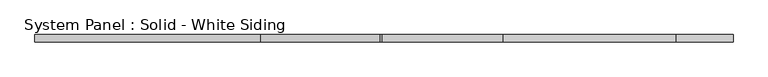
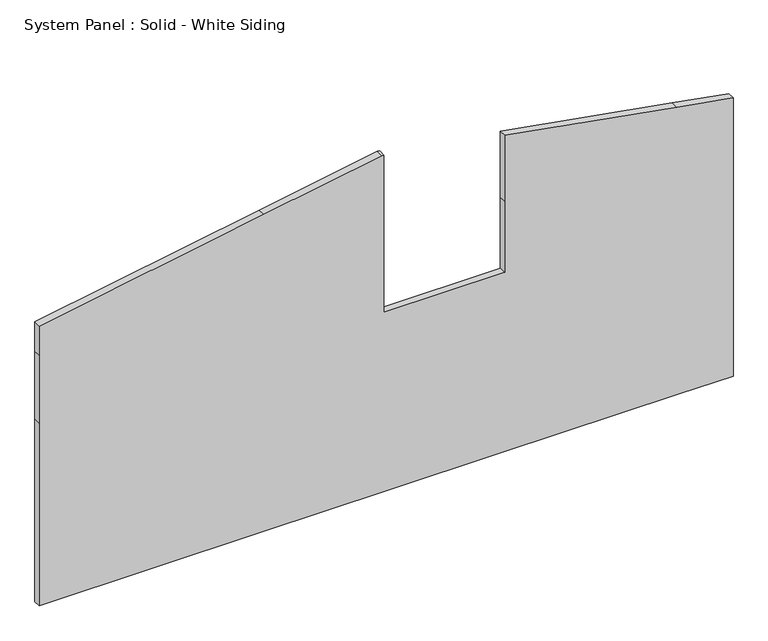
"""IFC4 building model written with IfcOpenShell, lengths in millimetres: plate geometry, System Panel : Solid - White Siding."""

from ifc_helpers import new_model, si_unit, frame, origin, place, context, project, spatial, polyline, outline, extrude, source, transform, mapped, element, save


def system_panel_solid_white_siding_d1a1bcec(model_context):
    return source(origin(), model_context, "Body", "SweptSolid", [
        extrude(outline(polyline([(0.0, -2959.1), (0.0, -1055.3257062), (0.0, 12.7), (0.0, 979.1257062), (0.0, 2489.2), (0.0, 2959.1), (1647.8580051, 2959.1), (2257.4580051, 2959.1), (2508.9751785, 2959.1), (2593.7755243, 2478.1733407), (2852.499686, 1010.8757062), (2257.4580051, 1010.8757062), (1616.1080051, 1010.8757062), (1616.1080051, -19.05), (2257.4580051, -19.05), (3034.1033761, -19.05), (3037.4624051, -38.1), (2860.0423651, -1044.2990469), (2522.4112944, -2959.1), (2257.4580051, -2959.1), (1647.8580051, -2959.1), (0.0, -2959.1)])), frame((0.0, -44.45, 0.0), z_axis=(0.0, 1.0, 0.0), x_axis=(0.0, 0.0, 1.0)), (0.0, 0.0, 1.0), 63.5),
    ])


if __name__ == "__main__":
    model = new_model("IFC4")
    model_context = context("Model", 3, world=origin())
    ifc_project = project(units=[si_unit("LENGTHUNIT", "METRE", prefix="MILLI")], contexts=[model_context])
    site = spatial("IfcSite", under=ifc_project)
    building = spatial("IfcBuilding", under=site)
    placement = place(None, origin())
    system_panel_solid_white_siding_shape = system_panel_solid_white_siding_d1a1bcec(model_context)
    element("IfcPlate", 1, ObjectType="System Panel : Solid - White Siding", at=placement, inside=building, context=model_context, shape_type="MappedRepresentation", body=[
        mapped(system_panel_solid_white_siding_shape, transform((0.0, 0.0, 0.0), x_axis=(1.0, 0.0, 0.0), y_axis=(0.0, 1.0, 0.0), z_axis=(0.0, 0.0, 1.0))),
    ])
    save(model, "model.ifc")

# Revit data of these elements
# Element 1 (IfcPlate, "System Panel : Solid - White Siding")
#   Materials on its faces: "White Siding"
# Materials
#   "White Siding": class "Unassigned", colour RGB 255 255 255, transparency 0
